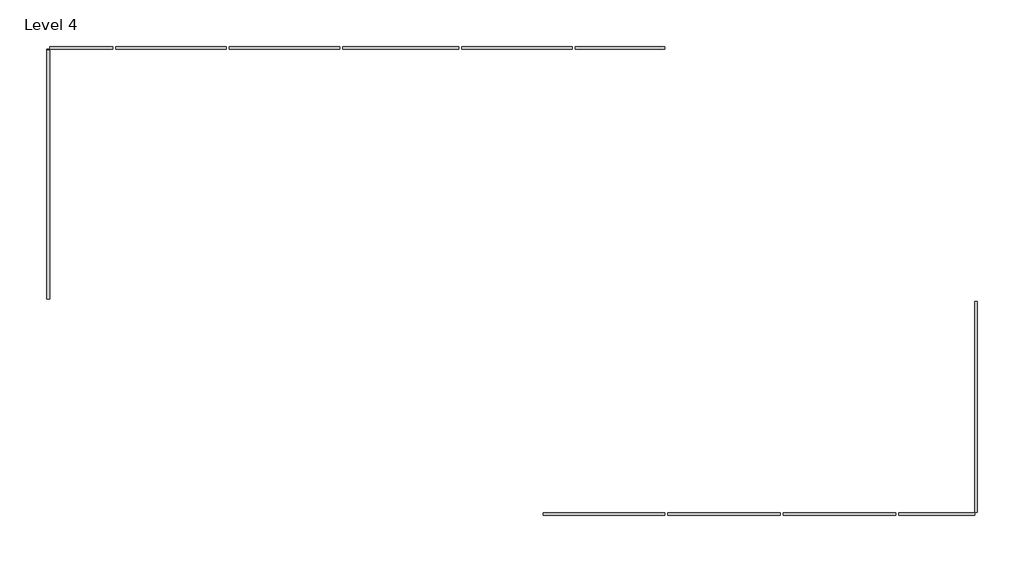
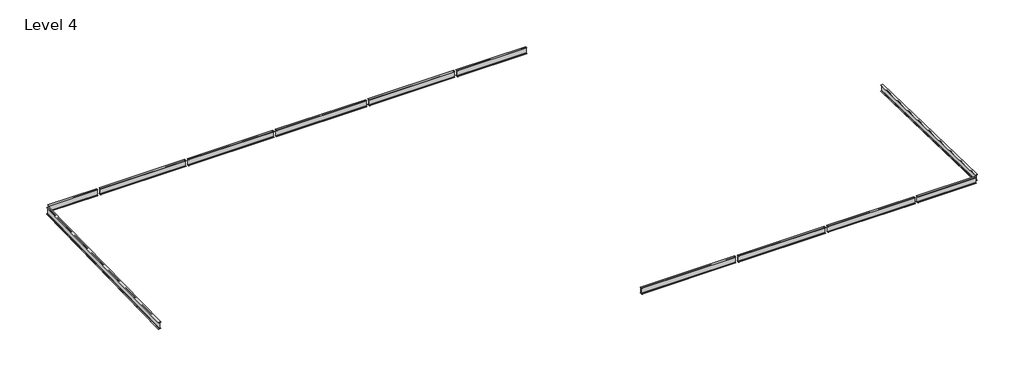
# One storey: 12 beams.
"""IFC4 building model written with IfcOpenShell, lengths in millimetres."""

import ifcopenshell
import ifcopenshell.guid

model = None  # the IFC model being written
_history = None  # IfcOwnerHistory: only IFC2X3 demands one
_inside = {}  # id of a spatial element -> (the spatial element, [elements in it])
_under = {}  # id of a project, library or spatial element -> (it, [spatial elements below it])
_declared = {}  # id of a project -> (the project, [libraries it declares])
_typed = {}  # id of a type object -> (the type object, [elements of that type])
_made_of = {}  # id of a material, layer set ... -> (it, [elements and type objects made of it])


def new_model(schema):
    """Start an empty IFC model of exactly this schema.

    Asked for "IFC4X3", IfcOpenShell would pick the latest addendum, in which some entities
    have other attributes; the version numbers below select the first issue.
    IFC2X3 requires an IfcOwnerHistory on every rooted entity: one is made here for all.
    """
    global model, _history
    if schema == "IFC4X3":
        model = ifcopenshell.file(schema_version=(4, 3, 0, 0))
    else:
        model = ifcopenshell.file(schema=schema)
    _inside.clear()
    _under.clear()
    _declared.clear()
    _typed.clear()
    _made_of.clear()
    _history = None
    if model.schema == "IFC2X3":
        org = make("IfcOrganization", Name="unknown")
        user = make(
            "IfcPersonAndOrganization",
            ThePerson=make("IfcPerson", FamilyName="unknown"),
            TheOrganization=org,
        )
        app = make(
            "IfcApplication",
            ApplicationDeveloper=org,
            Version="unknown",
            ApplicationFullName="unknown",
            ApplicationIdentifier="unknown",
        )
        _history = make(
            "IfcOwnerHistory",
            OwningUser=user,
            OwningApplication=app,
            ChangeAction="ADDED",
            CreationDate=0,
        )
    return model


def make(cls, **values):
    """One entity of the class cls with the attributes given. An attribute that is None is left unset."""
    return model.create_entity(
        cls, **{name: value for name, value in values.items() if value is not None}
    )


def rooted(cls, **values):
    """An entity with a GlobalId (a new one), such as an element, a storey or a relation."""
    return make(cls, GlobalId=ifcopenshell.guid.new(), OwnerHistory=_history, **values)


def si_unit(unit_type, name, prefix=None):
    """IfcSIUnit, for example si_unit("LENGTHUNIT", "METRE", prefix="MILLI")."""
    return make("IfcSIUnit", UnitType=unit_type, Prefix=prefix, Name=name)


def assignment(units):
    """IfcUnitAssignment: the units of a project."""
    return None if units is None else make("IfcUnitAssignment", Units=units)


def point(xyz):
    """IfcCartesianPoint."""
    return None if xyz is None else make("IfcCartesianPoint", Coordinates=xyz)


def direction(xyz):
    """IfcDirection."""
    return None if xyz is None else make("IfcDirection", DirectionRatios=xyz)


def frame(location, z_axis=None, x_axis=None):
    """IfcAxis2Placement3D, a coordinate frame: its origin and axes. An axis left out is left unset."""
    return make(
        "IfcAxis2Placement3D",
        Location=point(location),
        Axis=direction(z_axis),
        RefDirection=direction(x_axis),
    )


def frame_2d(location, x_axis=None):
    """IfcAxis2Placement2D, a coordinate frame in the plane: its origin and x axis."""
    return make(
        "IfcAxis2Placement2D", Location=point(location), RefDirection=direction(x_axis)
    )


def origin():
    """The frame at (0, 0, 0) with its axes left unset."""
    return frame((0.0, 0.0, 0.0))


def place(relative_to, where):
    """IfcLocalPlacement: puts the frame where relative to a parent placement (None: the world)."""
    return make(
        "IfcLocalPlacement", PlacementRelTo=relative_to, RelativePlacement=where
    )


def context(
    kind, dimensions, precision=None, world=None, true_north=None, identifier=None
):
    """IfcGeometricRepresentationContext, for example the 3D "Model" context."""
    return make(
        "IfcGeometricRepresentationContext",
        ContextIdentifier=identifier,
        ContextType=kind,
        CoordinateSpaceDimension=dimensions,
        Precision=precision,
        WorldCoordinateSystem=world,
        TrueNorth=true_north,
    )


def project(units=None, contexts=None):
    """IfcProject with its units and contexts."""
    return rooted(
        "IfcProject",
        Name="project",
        RepresentationContexts=contexts,
        UnitsInContext=assignment(units),
    )


def spatial(cls, under=None, at=None, **own):
    """A site, building, storey or space (cls), placed at a placement, below another one or the project."""
    s = rooted(cls, ObjectPlacement=at, **own)
    if under is not None:
        _under.setdefault(under.id(), (under, []))[1].append(s)
    return s


def polyline(points):
    """IfcPolyline through the points."""
    return make("IfcPolyline", Points=[point(p) for p in points])


def circle_curve(where, radius):
    """IfcCircle in the frame where."""
    return make("IfcCircle", Position=where, Radius=radius)


def trimmed(basis, trim1, trim2, sense, master):
    """IfcTrimmedCurve: the piece of a basis curve between two trims."""
    return make(
        "IfcTrimmedCurve",
        BasisCurve=basis,
        Trim1=trim1,
        Trim2=trim2,
        SenseAgreement=sense,
        MasterRepresentation=master,
    )


def segment(curve, same_sense, transition):
    """IfcCompositeCurveSegment."""
    return make(
        "IfcCompositeCurveSegment",
        Transition=transition,
        SameSense=same_sense,
        ParentCurve=curve,
    )


def composite_curve(segments, self_intersect=None):
    """IfcCompositeCurve: segments joined end to end."""
    return make("IfcCompositeCurve", Segments=segments, SelfIntersect=self_intersect)


def outline(outer, holes=None, kind="AREA"):
    """IfcArbitraryClosedProfileDef: a profile drawn as a closed curve; with holes, ...WithVoids."""
    if holes is None:
        return make("IfcArbitraryClosedProfileDef", ProfileType=kind, OuterCurve=outer)
    return make(
        "IfcArbitraryProfileDefWithVoids",
        ProfileType=kind,
        OuterCurve=outer,
        InnerCurves=holes,
    )


def extrude(swept, where, along, depth):
    """IfcExtrudedAreaSolid: the profile swept, set in the frame where, extruded along a direction by depth."""
    return make(
        "IfcExtrudedAreaSolid",
        SweptArea=swept,
        Position=where,
        ExtrudedDirection=direction(along),
        Depth=depth,
    )


def shape(context_of_items, identifier, shape_type, items):
    """IfcShapeRepresentation: the items that make up one representation, for example the "Body"."""
    return make(
        "IfcShapeRepresentation",
        ContextOfItems=context_of_items,
        RepresentationIdentifier=identifier,
        RepresentationType=shape_type,
        Items=items,
    )


def source(mapping_origin, context_of_items, identifier, shape_type, items):
    """IfcRepresentationMap: a shape defined once, which mapped items show again and again."""
    return make(
        "IfcRepresentationMap",
        MappingOrigin=mapping_origin,
        MappedRepresentation=shape(context_of_items, identifier, shape_type, items),
    )


def transform(
    local_origin,
    x_axis=None,
    y_axis=None,
    z_axis=None,
    scale=None,
    scale2=None,
    scale3=None,
    uniform=True,
):
    """IfcCartesianTransformationOperator3D, or its non-uniform kind. x_axis, y_axis, z_axis: its Axis1, 2, 3."""
    if uniform:
        return make(
            "IfcCartesianTransformationOperator3D",
            Axis1=direction(x_axis),
            Axis2=direction(y_axis),
            LocalOrigin=point(local_origin),
            Scale=scale,
            Axis3=direction(z_axis),
        )
    return make(
        "IfcCartesianTransformationOperator3DnonUniform",
        Axis1=direction(x_axis),
        Axis2=direction(y_axis),
        LocalOrigin=point(local_origin),
        Scale=scale,
        Axis3=direction(z_axis),
        Scale2=scale2,
        Scale3=scale3,
    )


def mapped(mapping_source, mapping_target):
    """IfcMappedItem: shows the shape of a source again, moved by a transform."""
    return make(
        "IfcMappedItem", MappingSource=mapping_source, MappingTarget=mapping_target
    )


def made_of(thing, what):
    """Note that an element or type object is made of a material, layer set ...; save() writes the relation."""
    if what is not None:
        _made_of.setdefault(what.id(), (what, []))[1].append(thing)
    return thing


def element(
    cls,
    number,
    at=None,
    inside=None,
    cuts=None,
    type_object=None,
    material=None,
    context=None,
    identifier="Body",
    shape_type=None,
    held_by="IfcProductDefinitionShape",
    body=None,
    shapes=None,
    **own,
):
    """One element of the class cls, such as IfcWall. Its Tag is "e" and its number.

    at: its placement. inside: the storey or other place that contains it. cuts: it is an
    opening in that element (IfcRelVoidsElement). A single representation is given by context,
    identifier, shape_type and body (its items); several are given by shapes. held_by: the class
    of the entity that holds the representations. save() writes the other relations.
    """
    e = rooted(cls, Tag="e%d" % number, ObjectPlacement=at, **own)
    if body is not None:
        shapes = [shape(context, identifier, shape_type, body)]
    if shapes is not None:
        e.Representation = make(held_by, Representations=shapes)
    if inside is not None:
        _inside.setdefault(inside.id(), (inside, []))[1].append(e)
    if cuts is not None:
        rooted(
            "IfcRelVoidsElement", RelatingBuildingElement=cuts, RelatedOpeningElement=e
        )
    if type_object is not None:
        _typed.setdefault(type_object.id(), (type_object, []))[1].append(e)
    return made_of(e, material)


def aggregate(whole, parts):
    """IfcRelAggregates: a whole, such as a stair, and the parts it consists of."""
    return rooted("IfcRelAggregates", RelatingObject=whole, RelatedObjects=parts)


def save(model, path):
    """Write the relations noted so far, then the file.

    IfcRelAggregates (storeys below a building ...), IfcRelContainedInSpatialStructure (elements
    in a storey), IfcRelDefinesByType, IfcRelAssociatesMaterial and IfcRelDeclares: one each for
    every whole, place, type object, material and project.
    """
    for whole, parts in _under.values():
        aggregate(whole, parts)
    for where, things in _inside.values():
        rooted(
            "IfcRelContainedInSpatialStructure",
            RelatedElements=things,
            RelatingStructure=where,
        )
    for kind, things in _typed.values():
        rooted("IfcRelDefinesByType", RelatedObjects=things, RelatingType=kind)
    for what, things in _made_of.values():
        rooted("IfcRelAssociatesMaterial", RelatedObjects=things, RelatingMaterial=what)
    for by, libraries in _declared.values():
        rooted("IfcRelDeclares", RelatingContext=by, RelatedDefinitions=libraries)
    model.write(path)


def w_shapes_w16x26_33867d62(model_context):
    return source(origin(), model_context, "Body", "SweptSolid", [
        extrude(outline(composite_curve([segment(polyline([(69.85, -190.627), (69.85, -199.39), (-69.85, -199.39), (-69.85, -190.627), (-13.3858, -190.627)]), True, "CONTINUOUS"), segment(trimmed(circle_curve(frame_2d((-13.3858, -180.4162)), 10.2108), [point((-13.3858, -190.627))], [point((-3.175, -180.4162))], True, "CARTESIAN"), True, "CONTINUOUS"), segment(polyline([(-3.175, -180.4162), (-3.175, 180.4162)]), True, "CONTINUOUS"), segment(trimmed(circle_curve(frame_2d((-13.3858, 180.4162)), 10.2108), [point((-3.175, 180.4162))], [point((-13.3858, 190.627))], True, "CARTESIAN"), True, "CONTINUOUS"), segment(polyline([(-13.3858, 190.627), (-69.85, 190.627), (-69.85, 199.39), (69.85, 199.39), (69.85, 190.627), (13.3858, 190.627)]), True, "CONTINUOUS"), segment(trimmed(circle_curve(frame_2d((13.3858, 180.4162)), 10.2108), [point((13.3858, 190.627))], [point((3.175, 180.4162))], True, "CARTESIAN"), True, "CONTINUOUS"), segment(polyline([(3.175, 180.4162), (3.175, -180.4162)]), True, "CONTINUOUS"), segment(trimmed(circle_curve(frame_2d((13.3858, -180.4162)), 10.2108), [point((3.175, -180.4162))], [point((13.3858, -190.627))], True, "CARTESIAN"), True, "CONTINUOUS"), segment(polyline([(13.3858, -190.627), (69.85, -190.627)]), True, "CONTINUOUS")], self_intersect=False)), frame((-2819.4, 0.0, 0.0), z_axis=(1.0, 0.0, 0.0), x_axis=(0.0, 1.0, 0.0)), (0.0, 0.0, 1.0), 5638.8),
    ])


def w_shapes_w16x26_2c91abbe(model_context):
    return source(origin(), model_context, "Body", "SweptSolid", [
        extrude(outline(composite_curve([segment(polyline([(69.85, -190.627), (69.85, -199.39), (-69.85, -199.39), (-69.85, -190.627), (-13.3858, -190.627)]), True, "CONTINUOUS"), segment(trimmed(circle_curve(frame_2d((-13.3858, -180.4162)), 10.2108), [point((-13.3858, -190.627))], [point((-3.175, -180.4162))], True, "CARTESIAN"), True, "CONTINUOUS"), segment(polyline([(-3.175, -180.4162), (-3.175, 180.4162)]), True, "CONTINUOUS"), segment(trimmed(circle_curve(frame_2d((-13.3858, 180.4162)), 10.2108), [point((-3.175, 180.4162))], [point((-13.3858, 190.627))], True, "CARTESIAN"), True, "CONTINUOUS"), segment(polyline([(-13.3858, 190.627), (-69.85, 190.627), (-69.85, 199.39), (69.85, 199.39), (69.85, 190.627), (13.3858, 190.627)]), True, "CONTINUOUS"), segment(trimmed(circle_curve(frame_2d((13.3858, 180.4162)), 10.2108), [point((13.3858, 190.627))], [point((3.175, 180.4162))], True, "CARTESIAN"), True, "CONTINUOUS"), segment(polyline([(3.175, 180.4162), (3.175, -180.4162)]), True, "CONTINUOUS"), segment(trimmed(circle_curve(frame_2d((13.3858, -180.4162)), 10.2108), [point((3.175, -180.4162))], [point((13.3858, -190.627))], True, "CARTESIAN"), True, "CONTINUOUS"), segment(polyline([(13.3858, -190.627), (69.85, -190.627)]), True, "CONTINUOUS")], self_intersect=False)), frame((-1905.0, 0.0, 0.0), z_axis=(1.0, 0.0, 0.0), x_axis=(0.0, 1.0, 0.0)), (0.0, 0.0, 1.0), 3810.0),
    ])


def w_shapes_w16x26_047c9101(model_context):
    return source(origin(), model_context, "Body", "SweptSolid", [
        extrude(outline(composite_curve([segment(polyline([(69.85, -190.627), (69.85, -199.39), (-69.85, -199.39), (-69.85, -190.627), (-13.3858, -190.627)]), True, "CONTINUOUS"), segment(trimmed(circle_curve(frame_2d((-13.3858, -180.4162)), 10.2108), [point((-13.3858, -190.627))], [point((-3.175, -180.4162))], True, "CARTESIAN"), True, "CONTINUOUS"), segment(polyline([(-3.175, -180.4162), (-3.175, 180.4162)]), True, "CONTINUOUS"), segment(trimmed(circle_curve(frame_2d((-13.3858, 180.4162)), 10.2108), [point((-3.175, 180.4162))], [point((-13.3858, 190.627))], True, "CARTESIAN"), True, "CONTINUOUS"), segment(polyline([(-13.3858, 190.627), (-69.85, 190.627), (-69.85, 199.39), (69.85, 199.39), (69.85, 190.627), (13.3858, 190.627)]), True, "CONTINUOUS"), segment(trimmed(circle_curve(frame_2d((13.3858, 180.4162)), 10.2108), [point((13.3858, 190.627))], [point((3.175, 180.4162))], True, "CARTESIAN"), True, "CONTINUOUS"), segment(polyline([(3.175, 180.4162), (3.175, -180.4162)]), True, "CONTINUOUS"), segment(trimmed(circle_curve(frame_2d((13.3858, -180.4162)), 10.2108), [point((3.175, -180.4162))], [point((13.3858, -190.627))], True, "CARTESIAN"), True, "CONTINUOUS"), segment(polyline([(13.3858, -190.627), (69.85, -190.627)]), True, "CONTINUOUS")], self_intersect=False)), frame((-3048.0, 0.0, 0.0), z_axis=(1.0, 0.0, 0.0), x_axis=(0.0, 1.0, 0.0)), (0.0, 0.0, 1.0), 6096.0),
    ])


def w_shapes_w16x26_f77c1278(model_context):
    return source(origin(), model_context, "Body", "SweptSolid", [
        extrude(outline(composite_curve([segment(polyline([(69.85, -190.627), (69.85, -199.39), (-69.85, -199.39), (-69.85, -190.627), (-13.3858, -190.627)]), True, "CONTINUOUS"), segment(trimmed(circle_curve(frame_2d((-13.3858, -180.4162)), 10.2108), [point((-13.3858, -190.627))], [point((-3.175, -180.4162))], True, "CARTESIAN"), True, "CONTINUOUS"), segment(polyline([(-3.175, -180.4162), (-3.175, 180.4162)]), True, "CONTINUOUS"), segment(trimmed(circle_curve(frame_2d((-13.3858, 180.4162)), 10.2108), [point((-3.175, 180.4162))], [point((-13.3858, 190.627))], True, "CARTESIAN"), True, "CONTINUOUS"), segment(polyline([(-13.3858, 190.627), (-69.85, 190.627), (-69.85, 199.39), (69.85, 199.39), (69.85, 190.627), (13.3858, 190.627)]), True, "CONTINUOUS"), segment(trimmed(circle_curve(frame_2d((13.3858, 180.4162)), 10.2108), [point((13.3858, 190.627))], [point((3.175, 180.4162))], True, "CARTESIAN"), True, "CONTINUOUS"), segment(polyline([(3.175, 180.4162), (3.175, -180.4162)]), True, "CONTINUOUS"), segment(trimmed(circle_curve(frame_2d((13.3858, -180.4162)), 10.2108), [point((3.175, -180.4162))], [point((13.3858, -190.627))], True, "CARTESIAN"), True, "CONTINUOUS"), segment(polyline([(13.3858, -190.627), (69.85, -190.627)]), True, "CONTINUOUS")], self_intersect=False)), frame((-2921.0, 0.0, 0.0), z_axis=(1.0, 0.0, 0.0), x_axis=(0.0, 1.0, 0.0)), (0.0, 0.0, 1.0), 5842.0),
    ])


def w_shapes_w16x26_29ee5571(model_context):
    return source(origin(), model_context, "Body", "SweptSolid", [
        extrude(outline(composite_curve([segment(polyline([(69.85, -190.627), (69.85, -199.39), (-69.85, -199.39), (-69.85, -190.627), (-13.3858, -190.627)]), True, "CONTINUOUS"), segment(trimmed(circle_curve(frame_2d((-13.3858, -180.4162)), 10.2108), [point((-13.3858, -190.627))], [point((-3.175, -180.4162))], True, "CARTESIAN"), True, "CONTINUOUS"), segment(polyline([(-3.175, -180.4162), (-3.175, 180.4162)]), True, "CONTINUOUS"), segment(trimmed(circle_curve(frame_2d((-13.3858, 180.4162)), 10.2108), [point((-3.175, 180.4162))], [point((-13.3858, 190.627))], True, "CARTESIAN"), True, "CONTINUOUS"), segment(polyline([(-13.3858, 190.627), (-69.85, 190.627), (-69.85, 199.39), (69.85, 199.39), (69.85, 190.627), (13.3858, 190.627)]), True, "CONTINUOUS"), segment(trimmed(circle_curve(frame_2d((13.3858, 180.4162)), 10.2108), [point((13.3858, 190.627))], [point((3.175, 180.4162))], True, "CARTESIAN"), True, "CONTINUOUS"), segment(polyline([(3.175, 180.4162), (3.175, -180.4162)]), True, "CONTINUOUS"), segment(trimmed(circle_curve(frame_2d((13.3858, -180.4162)), 10.2108), [point((3.175, -180.4162))], [point((13.3858, -190.627))], True, "CARTESIAN"), True, "CONTINUOUS"), segment(polyline([(13.3858, -190.627), (69.85, -190.627)]), True, "CONTINUOUS")], self_intersect=False)), frame((-2768.6, 0.0, 0.0), z_axis=(1.0, 0.0, 0.0), x_axis=(0.0, 1.0, 0.0)), (0.0, 0.0, 1.0), 5537.2),
    ])


def w_shapes_w16x26_fcd2c860(model_context):
    return source(origin(), model_context, "Body", "SweptSolid", [
        extrude(outline(composite_curve([segment(polyline([(69.85, -190.627), (69.85, -199.39), (-69.85, -199.39), (-69.85, -190.627), (-13.3858, -190.627)]), True, "CONTINUOUS"), segment(trimmed(circle_curve(frame_2d((-13.3858, -180.4162)), 10.2108), [point((-13.3858, -190.627))], [point((-3.175, -180.4162))], True, "CARTESIAN"), True, "CONTINUOUS"), segment(polyline([(-3.175, -180.4162), (-3.175, 180.4162)]), True, "CONTINUOUS"), segment(trimmed(circle_curve(frame_2d((-13.3858, 180.4162)), 10.2108), [point((-3.175, 180.4162))], [point((-13.3858, 190.627))], True, "CARTESIAN"), True, "CONTINUOUS"), segment(polyline([(-13.3858, 190.627), (-69.85, 190.627), (-69.85, 199.39), (69.85, 199.39), (69.85, 190.627), (13.3858, 190.627)]), True, "CONTINUOUS"), segment(trimmed(circle_curve(frame_2d((13.3858, 180.4162)), 10.2108), [point((13.3858, 190.627))], [point((3.175, 180.4162))], True, "CARTESIAN"), True, "CONTINUOUS"), segment(polyline([(3.175, 180.4162), (3.175, -180.4162)]), True, "CONTINUOUS"), segment(trimmed(circle_curve(frame_2d((13.3858, -180.4162)), 10.2108), [point((3.175, -180.4162))], [point((13.3858, -190.627))], True, "CARTESIAN"), True, "CONTINUOUS"), segment(polyline([(13.3858, -190.627), (69.85, -190.627)]), True, "CONTINUOUS")], self_intersect=False)), frame((-1587.5, 0.0, 0.0), z_axis=(1.0, 0.0, 0.0), x_axis=(0.0, 1.0, 0.0)), (0.0, 0.0, 1.0), 3175.0),
    ])


def w_shapes_w16x26_d059226d(model_context):
    return source(origin(), model_context, "Body", "SweptSolid", [
        extrude(outline(composite_curve([segment(polyline([(69.85, -190.627), (69.85, -199.39), (-69.85, -199.39), (-69.85, -190.627), (-13.3858, -190.627)]), True, "CONTINUOUS"), segment(trimmed(circle_curve(frame_2d((-13.3858, -180.4162)), 10.2108), [point((-13.3858, -190.627))], [point((-3.175, -180.4162))], True, "CARTESIAN"), True, "CONTINUOUS"), segment(polyline([(-3.175, -180.4162), (-3.175, 180.4162)]), True, "CONTINUOUS"), segment(trimmed(circle_curve(frame_2d((-13.3858, 180.4162)), 10.2108), [point((-3.175, 180.4162))], [point((-13.3858, 190.627))], True, "CARTESIAN"), True, "CONTINUOUS"), segment(polyline([(-13.3858, 190.627), (-69.85, 190.627), (-69.85, 199.39), (69.85, 199.39), (69.85, 190.627), (13.3858, 190.627)]), True, "CONTINUOUS"), segment(trimmed(circle_curve(frame_2d((13.3858, 180.4162)), 10.2108), [point((13.3858, 190.627))], [point((3.175, 180.4162))], True, "CARTESIAN"), True, "CONTINUOUS"), segment(polyline([(3.175, 180.4162), (3.175, -180.4162)]), True, "CONTINUOUS"), segment(trimmed(circle_curve(frame_2d((13.3858, -180.4162)), 10.2108), [point((3.175, -180.4162))], [point((13.3858, -190.627))], True, "CARTESIAN"), True, "CONTINUOUS"), segment(polyline([(13.3858, -190.627), (69.85, -190.627)]), True, "CONTINUOUS")], self_intersect=False)), frame((-2247.9, 0.0, 0.0), z_axis=(1.0, 0.0, 0.0), x_axis=(0.0, 1.0, 0.0)), (0.0, 0.0, 1.0), 4495.8),
    ])


def w_wide_flange_w16x26_a3dbe27b(model_context):
    return source(origin(), model_context, "Body", "SweptSolid", [
        extrude(outline(composite_curve([segment(polyline([(69.85, -190.627), (69.85, -199.39), (-69.85, -199.39), (-69.85, -190.627), (-21.3995, -190.627)]), True, "CONTINUOUS"), segment(trimmed(circle_curve(frame_2d((-21.3995, -172.4025)), 18.2245), [point((-21.3995, -190.627))], [point((-3.175, -172.4025))], True, "CARTESIAN"), True, "CONTINUOUS"), segment(polyline([(-3.175, -172.4025), (-3.175, 172.4025)]), True, "CONTINUOUS"), segment(trimmed(circle_curve(frame_2d((-21.3995, 172.4025)), 18.2245), [point((-3.175, 172.4025))], [point((-21.3995, 190.627))], True, "CARTESIAN"), True, "CONTINUOUS"), segment(polyline([(-21.3995, 190.627), (-69.85, 190.627), (-69.85, 199.39), (69.85, 199.39), (69.85, 190.627), (21.3995, 190.627)]), True, "CONTINUOUS"), segment(trimmed(circle_curve(frame_2d((21.3995, 172.4025)), 18.2245), [point((21.3995, 190.627))], [point((3.175, 172.4025))], True, "CARTESIAN"), True, "CONTINUOUS"), segment(polyline([(3.175, 172.4025), (3.175, -172.4025)]), True, "CONTINUOUS"), segment(trimmed(circle_curve(frame_2d((21.3995, -172.4025)), 18.2245), [point((3.175, -172.4025))], [point((21.3995, -190.627))], True, "CARTESIAN"), True, "CONTINUOUS"), segment(polyline([(21.3995, -190.627), (69.85, -190.627)]), True, "CONTINUOUS")], self_intersect=False)), frame((-5304.0661233, 0.0, 0.0), z_axis=(1.0, 0.0, 0.0), x_axis=(0.0, 1.0, 0.0)), (0.0, 0.0, 1.0), 10591.3863205),
    ])


def w_wide_flange_w18x35_dd771225(model_context):
    return source(origin(), model_context, "Body", "SweptSolid", [
        extrude(outline(composite_curve([segment(polyline([(76.2, -213.995), (76.2, -224.79), (-76.2, -224.79), (-76.2, -213.995), (-21.59, -213.995)]), True, "CONTINUOUS"), segment(trimmed(circle_curve(frame_2d((-21.59, -196.215)), 17.78), [point((-21.59, -213.995))], [point((-3.81, -196.215))], True, "CARTESIAN"), True, "CONTINUOUS"), segment(polyline([(-3.81, -196.215), (-3.81, 196.215)]), True, "CONTINUOUS"), segment(trimmed(circle_curve(frame_2d((-21.59, 196.215)), 17.78), [point((-3.81, 196.215))], [point((-21.59, 213.995))], True, "CARTESIAN"), True, "CONTINUOUS"), segment(polyline([(-21.59, 213.995), (-76.2, 213.995), (-76.2, 224.79), (76.2, 224.79), (76.2, 213.995), (21.59, 213.995)]), True, "CONTINUOUS"), segment(trimmed(circle_curve(frame_2d((21.59, 196.215)), 17.78), [point((21.59, 213.995))], [point((3.81, 196.215))], True, "CARTESIAN"), True, "CONTINUOUS"), segment(polyline([(3.81, 196.215), (3.81, -196.215)]), True, "CONTINUOUS"), segment(trimmed(circle_curve(frame_2d((21.59, -196.215)), 17.78), [point((3.81, -196.215))], [point((21.59, -213.995))], True, "CARTESIAN"), True, "CONTINUOUS"), segment(polyline([(21.59, -213.995), (76.2, -213.995)]), True, "CONTINUOUS")], self_intersect=False)), frame((-6252.7104992, 0.0, 0.0), z_axis=(1.0, 0.0, 0.0), x_axis=(0.0, 1.0, 0.0)), (0.0, 0.0, 1.0), 12523.1165167),
    ])


model = new_model("IFC4")

# Units and contexts
model_context = context("Model", 3, world=origin())
ifc_project = project(units=[si_unit("LENGTHUNIT", "METRE", prefix="MILLI")], contexts=[model_context])

# Site, building, storey
site = spatial("IfcSite", under=ifc_project)
building = spatial("IfcBuilding", under=site)
storey = spatial("IfcBuildingStorey", under=building, Name="Level 4", Elevation=12547.6)

# Beams
placement = place(None, origin())
w_shapes_w16x26_shape = w_shapes_w16x26_33867d62(model_context)
element("IfcBeam", 1, ObjectType="W Shapes : W16X26", at=placement, inside=storey, context=model_context, shape_type="MappedRepresentation", body=[
    mapped(w_shapes_w16x26_shape, transform((9176.4325311, -14300.0323339, 12284.71), x_axis=(-1.0, 0.0, 0.0), y_axis=(0.0, -1.0, 0.0), z_axis=(0.0, 0.0, 1.0))),
])
element("IfcBeam", 2, ObjectType="W Shapes : W16X26", at=placement, inside=storey, context=model_context, shape_type="MappedRepresentation", body=[
    mapped(w_shapes_w16x26_shape, transform((3385.2325311, -14300.0323339, 12284.71), x_axis=(-1.0, 0.0, 0.0), y_axis=(0.0, -1.0, 0.0), z_axis=(0.0, 0.0, 1.0))),
])
w_shapes_w16x26_2_shape = w_shapes_w16x26_2c91abbe(model_context)
element("IfcBeam", 3, ObjectType="W Shapes : W16X26", at=placement, inside=storey, context=model_context, shape_type="MappedRepresentation", body=[
    mapped(w_shapes_w16x26_2_shape, transform((14053.2325311, -14300.0323339, 12284.71), x_axis=(-1.0, 0.0, 0.0), y_axis=(0.0, -1.0, 0.0), z_axis=(0.0, 0.0, 1.0))),
])
w_shapes_w16x26_3_shape = w_shapes_w16x26_047c9101(model_context)
element("IfcBeam", 4, ObjectType="W Shapes : W16X26", at=placement, inside=storey, context=model_context, shape_type="MappedRepresentation", body=[
    mapped(w_shapes_w16x26_3_shape, transform((-2634.5674689, -14300.0323339, 12284.71), x_axis=(-1.0, 0.0, 0.0), y_axis=(0.0, -1.0, 0.0), z_axis=(0.0, 0.0, 1.0))),
])
w_shapes_w16x26_4_shape = w_shapes_w16x26_f77c1278(model_context)
element("IfcBeam", 5, ObjectType="W Shapes : W16X26", at=placement, inside=storey, context=model_context, shape_type="MappedRepresentation", body=[
    mapped(w_shapes_w16x26_4_shape, transform((-12845.3674689, 9118.7676661, 12386.31), x_axis=(-1.0, 0.0, 0.0), y_axis=(0.0, -1.0, 0.0), z_axis=(0.0, 0.0, 1.0))),
])
w_shapes_w16x26_5_shape = w_shapes_w16x26_29ee5571(model_context)
element("IfcBeam", 6, ObjectType="W Shapes : W16X26", at=placement, inside=storey, context=model_context, shape_type="MappedRepresentation", body=[
    mapped(w_shapes_w16x26_5_shape, transform((-24376.9674689, 9118.7676661, 12386.31), x_axis=(-1.0, 0.0, 0.0), y_axis=(0.0, -1.0, 0.0), z_axis=(0.0, 0.0, 1.0))),
])
element("IfcBeam", 7, ObjectType="W Shapes : W16X26", at=placement, inside=storey, context=model_context, shape_type="MappedRepresentation", body=[
    mapped(w_shapes_w16x26_5_shape, transform((-18687.3674689, 9118.7676661, 12386.31), x_axis=(-1.0, 0.0, 0.0), y_axis=(0.0, -1.0, 0.0), z_axis=(0.0, 0.0, 1.0))),
])
element("IfcBeam", 8, ObjectType="W Shapes : W16X26", at=placement, inside=storey, context=model_context, shape_type="MappedRepresentation", body=[
    mapped(w_shapes_w16x26_5_shape, transform((-7003.3674689, 9118.7676661, 12386.31), x_axis=(-1.0, 0.0, 0.0), y_axis=(0.0, -1.0, 0.0), z_axis=(0.0, 0.0, 1.0))),
])
w_shapes_w16x26_6_shape = w_shapes_w16x26_fcd2c860(model_context)
element("IfcBeam", 9, ObjectType="W Shapes : W16X26", at=placement, inside=storey, context=model_context, shape_type="MappedRepresentation", body=[
    mapped(w_shapes_w16x26_6_shape, transform((-28885.4674689, 9118.7676661, 12386.31), x_axis=(-1.0, 0.0, 0.0), y_axis=(0.0, -1.0, 0.0), z_axis=(0.0, 0.0, 1.0))),
])
w_shapes_w16x26_7_shape = w_shapes_w16x26_d059226d(model_context)
element("IfcBeam", 10, ObjectType="W Shapes : W16X26", at=placement, inside=storey, context=model_context, shape_type="MappedRepresentation", body=[
    mapped(w_shapes_w16x26_7_shape, transform((-1834.4674689, 9118.7676661, 12386.31), x_axis=(-1.0, 0.0, 0.0), y_axis=(0.0, -1.0, 0.0), z_axis=(0.0, 0.0, 1.0))),
])
w_wide_flange_w16x26_shape = w_wide_flange_w16x26_a3dbe27b(model_context)
element("IfcBeam", 11, ObjectType="W-Wide Flange : W16X26", at=placement, inside=storey, context=model_context, shape_type="MappedRepresentation", body=[
    mapped(w_wide_flange_w16x26_shape, transform((16034.4325311, -8933.1156644, 12208.5773842), x_axis=(0.0, -0.9996620484514823, 0.025995939794247025), y_axis=(1.0, 0.0, 0.0), z_axis=(0.0, 0.02599593979424703, 0.9996620484514824))),
])
w_wide_flange_w18x35_shape = w_wide_flange_w18x35_dd771225(model_context)
element("IfcBeam", 12, ObjectType="W-Wide Flange : W18X35", at=placement, inside=storey, context=model_context, shape_type="MappedRepresentation", body=[
    mapped(w_wide_flange_w18x35_shape, transform((-30549.1674689, 2786.4217531, 12183.1645975), x_axis=(0.0, -0.9997571176046883, -0.022038734055413938), y_axis=(1.0, 0.0, 0.0), z_axis=(0.0, -0.022038734055413938, 0.9997571176046884))),
])

save(model, "model.ifc")

# Revit data of these elements
# Type "W Shapes : W16X26"
#   Section Name Key = "W16x26"
#   Assembly Code = "B10"
#   Width = 5.500"
#   Web Thickness = 0.250"
#   Web Fillet = 0.402"
#   Warping Constant = 565.00 in⁶
#   Torsional Moment of Inertia = 0.262 in⁴
#   Section Area = 7.68 in²
#   Plastic Modulus weak axis = 5.48 in³
#   Plastic Modulus strong axis = 44.20 in³
#   Perimeter = 4.35 ft²/ft
#   Nominal Weight = 26.00 lbf/ft
#   Moment of Inertia weak axis = 9.59 in⁴
#   Moment of Inertia strong axis = 301.00 in⁴
#   Height = 15.700"
#   Flange Thickness = 0.345"
#   Elastic Modulus weak axis = 3.49 in³
#   Elastic Modulus strong axis = 38.40 in³
#   Centroid Vertical = 7.850"
#   Centroid Horizontal = 2.750"
#   Bolt Spacing = 0' - 3 1/2"
#   Length [instance default] = 5' - 0"
#   Structural Material [instance default] = Steel ASTM A992
#   Principal Axes Angle = 0
# Type "W-Wide Flange : W16X26"
#   Assembly Code = "B10"
#   W = 26
#   Length [instance default] = 5' - 0"
#   bf = 0' - 5 1/2"
#   d = 1' - 3.7"
#   k = 0' - 1 1/16"
#   k2 = 0' - 0.7175"
#   tf = 0' - 0.345"
#   tw = 0' - 0 1/4"
#   A = 0.0533333 SF
#   Structural Material [instance default] = Steel ASTM A992
# Type "W-Wide Flange : W18X35"
#   Assembly Code = "B10"
#   W = 35
#   Length [instance default] = 5' - 0"
#   bf = 0' - 6"
#   d = 1' - 5.7"
#   k = 0' - 1 1/8"
#   k2 = 0' - 0.7"
#   tf = 0' - 0.425"
#   tw = 0' - 0.3"
#   A = 0.0715278 SF
#   Structural Material [instance default] = Steel ASTM A992
# Elements 1, 2, 3, 4, 5, 6, 7, 8, 9, 10 (IfcBeam, "W Shapes : W16X26")
#   Comments = ""
#   Structural Material = Steel ASTM A36
#   Phase Created = New Construction
#   Materials on its faces: "Steel ASTM A36"
# Element 11 (IfcBeam, "W-Wide Flange : W16X26")
#   Comments = ""
#   Structural Material = Steel ASTM A36
#   Phase Created = New Construction
#   Materials on its faces: "Steel ASTM A36"
# Element 12 (IfcBeam, "W-Wide Flange : W18X35")
#   Comments = ""
#   Structural Material = Steel ASTM A36
#   Phase Created = New Construction
#   Materials on its faces: "Steel ASTM A36"
# Materials
#   "Steel ASTM A992": class "Metal", colour RGB 199 199 199, transparency 0, Description = "Structural steel 50ksi", Cost = 0
#   "Steel ASTM A36": class "Metal", colour RGB 199 199 199, transparency 0, Description = "Structural steel, ASTM A36 Grade B, mill finish", Cost = 0
